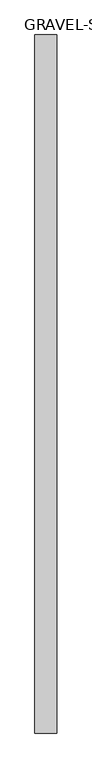
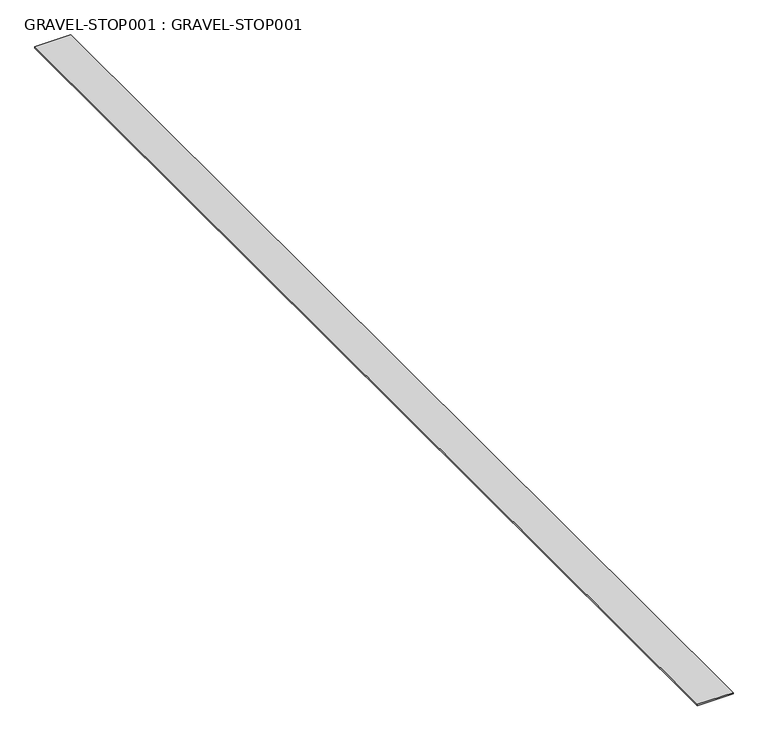
"""IFC4 building model written with IfcOpenShell, lengths in millimetres: proxy geometry, GRAVEL-STOP001 : GRAVEL-STOP001."""

from ifc_helpers import new_model, si_unit, frame, origin, place, context, project, spatial, polyline, outline, extrude, source, transform, mapped, element, save


def gravel_stop001_gravel_stop001_5ee6ed41(model_context):
    return source(origin(), model_context, "Body", "SweptSolid", [
        extrude(outline(polyline([(-4968.0627753, 947.3593427), (-4905.7346672, 947.3593427), (-4905.7346672, -1052.8906573), (-4968.0627753, -1052.8906573), (-4968.0627753, 947.3593427)])), frame((0.0, 0.0, 40252.8572765), z_axis=(0.0, 0.0, 1.0), x_axis=(1.0, 0.0, 0.0)), (0.0, 0.0, 1.0), 2.3397091),
    ])


if __name__ == "__main__":
    model = new_model("IFC4")
    model_context = context("Model", 3, world=origin())
    ifc_project = project(units=[si_unit("LENGTHUNIT", "METRE", prefix="MILLI")], contexts=[model_context])
    site = spatial("IfcSite", under=ifc_project)
    building = spatial("IfcBuilding", under=site)
    placement = place(None, origin())
    gravel_stop001_gravel_stop001_shape = gravel_stop001_gravel_stop001_5ee6ed41(model_context)
    element("IfcBuildingElementProxy", 1, Name="GRAVEL-STOP001 : GRAVEL-STOP001", ObjectType="GRAVEL-STOP001 : GRAVEL-STOP001", at=placement, inside=building, context=model_context, shape_type="MappedRepresentation", body=[
        mapped(gravel_stop001_gravel_stop001_shape, transform((0.0, 0.0, 0.0), x_axis=(1.0, 0.0, 0.0), y_axis=(0.0, 1.0, 0.0), z_axis=(0.0, 0.0, 1.0))),
    ])
    save(model, "model.ifc")

# Revit data of these elements
# Type "GRAVEL-STOP001 : GRAVEL-STOP001"
#   NameOverride = "GRAVEL-STOP001"
# Element 1 (IfcBuildingElementProxy, "GRAVEL-STOP001 : GRAVEL-STOP001")
#   Materials on its faces: "METAL FLASHING"
# Materials
#   "METAL FLASHING": class "Unassigned", colour RGB 128 128 128, transparency 0
